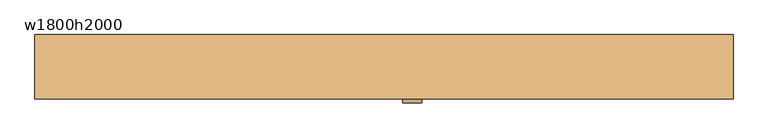
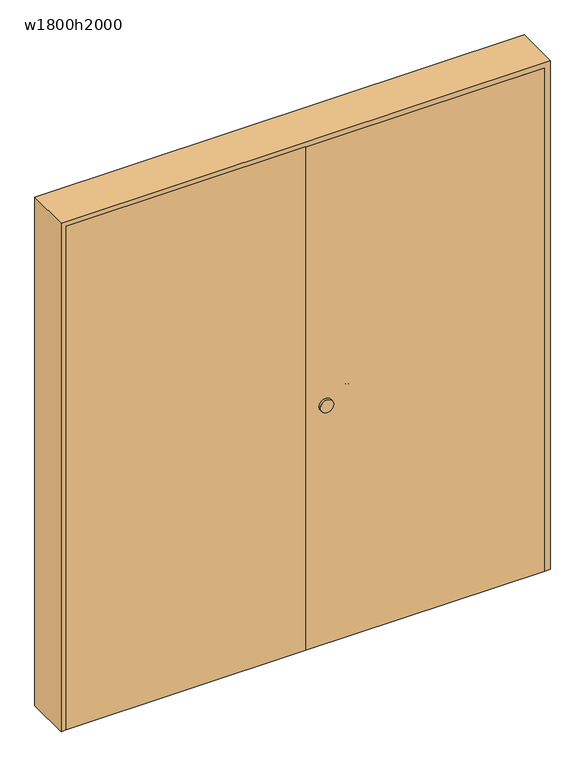
"""IFC4 building model written with IfcOpenShell, lengths in millimetres: door geometry, 二重 : w1800h2000."""

import ifcopenshell
import ifcopenshell.guid

model = None  # the IFC model being written
_history = None  # IfcOwnerHistory: only IFC2X3 demands one
_inside = {}  # id of a spatial element -> (the spatial element, [elements in it])
_under = {}  # id of a project, library or spatial element -> (it, [spatial elements below it])
_declared = {}  # id of a project -> (the project, [libraries it declares])
_typed = {}  # id of a type object -> (the type object, [elements of that type])
_made_of = {}  # id of a material, layer set ... -> (it, [elements and type objects made of it])


def new_model(schema):
    """Start an empty IFC model of exactly this schema.

    Asked for "IFC4X3", IfcOpenShell would pick the latest addendum, in which some entities
    have other attributes; the version numbers below select the first issue.
    IFC2X3 requires an IfcOwnerHistory on every rooted entity: one is made here for all.
    """
    global model, _history
    if schema == "IFC4X3":
        model = ifcopenshell.file(schema_version=(4, 3, 0, 0))
    else:
        model = ifcopenshell.file(schema=schema)
    _inside.clear()
    _under.clear()
    _declared.clear()
    _typed.clear()
    _made_of.clear()
    _history = None
    if model.schema == "IFC2X3":
        org = make("IfcOrganization", Name="unknown")
        user = make(
            "IfcPersonAndOrganization",
            ThePerson=make("IfcPerson", FamilyName="unknown"),
            TheOrganization=org,
        )
        app = make(
            "IfcApplication",
            ApplicationDeveloper=org,
            Version="unknown",
            ApplicationFullName="unknown",
            ApplicationIdentifier="unknown",
        )
        _history = make(
            "IfcOwnerHistory",
            OwningUser=user,
            OwningApplication=app,
            ChangeAction="ADDED",
            CreationDate=0,
        )
    return model


def make(cls, **values):
    """One entity of the class cls with the attributes given. An attribute that is None is left unset."""
    return model.create_entity(
        cls, **{name: value for name, value in values.items() if value is not None}
    )


def rooted(cls, **values):
    """An entity with a GlobalId (a new one), such as an element, a storey or a relation."""
    return make(cls, GlobalId=ifcopenshell.guid.new(), OwnerHistory=_history, **values)


def si_unit(unit_type, name, prefix=None):
    """IfcSIUnit, for example si_unit("LENGTHUNIT", "METRE", prefix="MILLI")."""
    return make("IfcSIUnit", UnitType=unit_type, Prefix=prefix, Name=name)


def assignment(units):
    """IfcUnitAssignment: the units of a project."""
    return None if units is None else make("IfcUnitAssignment", Units=units)


def point(xyz):
    """IfcCartesianPoint."""
    return None if xyz is None else make("IfcCartesianPoint", Coordinates=xyz)


def direction(xyz):
    """IfcDirection."""
    return None if xyz is None else make("IfcDirection", DirectionRatios=xyz)


def frame(location, z_axis=None, x_axis=None):
    """IfcAxis2Placement3D, a coordinate frame: its origin and axes. An axis left out is left unset."""
    return make(
        "IfcAxis2Placement3D",
        Location=point(location),
        Axis=direction(z_axis),
        RefDirection=direction(x_axis),
    )


def frame_2d(location, x_axis=None):
    """IfcAxis2Placement2D, a coordinate frame in the plane: its origin and x axis."""
    return make(
        "IfcAxis2Placement2D", Location=point(location), RefDirection=direction(x_axis)
    )


def origin():
    """The frame at (0, 0, 0) with its axes left unset."""
    return frame((0.0, 0.0, 0.0))


def origin_with_axes():
    """The frame at (0, 0, 0) with the z axis (0, 0, 1) and the x axis (1, 0, 0) written out."""
    return frame((0.0, 0.0, 0.0), z_axis=(0.0, 0.0, 1.0), x_axis=(1.0, 0.0, 0.0))


def place(relative_to, where):
    """IfcLocalPlacement: puts the frame where relative to a parent placement (None: the world)."""
    return make(
        "IfcLocalPlacement", PlacementRelTo=relative_to, RelativePlacement=where
    )


def context(
    kind, dimensions, precision=None, world=None, true_north=None, identifier=None
):
    """IfcGeometricRepresentationContext, for example the 3D "Model" context."""
    return make(
        "IfcGeometricRepresentationContext",
        ContextIdentifier=identifier,
        ContextType=kind,
        CoordinateSpaceDimension=dimensions,
        Precision=precision,
        WorldCoordinateSystem=world,
        TrueNorth=true_north,
    )


def project(units=None, contexts=None):
    """IfcProject with its units and contexts."""
    return rooted(
        "IfcProject",
        Name="project",
        RepresentationContexts=contexts,
        UnitsInContext=assignment(units),
    )


def spatial(cls, under=None, at=None, **own):
    """A site, building, storey or space (cls), placed at a placement, below another one or the project."""
    s = rooted(cls, ObjectPlacement=at, **own)
    if under is not None:
        _under.setdefault(under.id(), (under, []))[1].append(s)
    return s


def polyline(points):
    """IfcPolyline through the points."""
    return make("IfcPolyline", Points=[point(p) for p in points])


def circle_curve(where, radius):
    """IfcCircle in the frame where."""
    return make("IfcCircle", Position=where, Radius=radius)


def ellipse_curve(where, semi_axis1, semi_axis2):
    """IfcEllipse in the frame where."""
    return make(
        "IfcEllipse", Position=where, SemiAxis1=semi_axis1, SemiAxis2=semi_axis2
    )


def trimmed(basis, trim1, trim2, sense, master):
    """IfcTrimmedCurve: the piece of a basis curve between two trims."""
    return make(
        "IfcTrimmedCurve",
        BasisCurve=basis,
        Trim1=trim1,
        Trim2=trim2,
        SenseAgreement=sense,
        MasterRepresentation=master,
    )


def segment(curve, same_sense, transition):
    """IfcCompositeCurveSegment."""
    return make(
        "IfcCompositeCurveSegment",
        Transition=transition,
        SameSense=same_sense,
        ParentCurve=curve,
    )


def composite_curve(segments, self_intersect=None):
    """IfcCompositeCurve: segments joined end to end."""
    return make("IfcCompositeCurve", Segments=segments, SelfIntersect=self_intersect)


def outline(outer, holes=None, kind="AREA"):
    """IfcArbitraryClosedProfileDef: a profile drawn as a closed curve; with holes, ...WithVoids."""
    if holes is None:
        return make("IfcArbitraryClosedProfileDef", ProfileType=kind, OuterCurve=outer)
    return make(
        "IfcArbitraryProfileDefWithVoids",
        ProfileType=kind,
        OuterCurve=outer,
        InnerCurves=holes,
    )


def extrude(swept, where, along, depth):
    """IfcExtrudedAreaSolid: the profile swept, set in the frame where, extruded along a direction by depth."""
    return make(
        "IfcExtrudedAreaSolid",
        SweptArea=swept,
        Position=where,
        ExtrudedDirection=direction(along),
        Depth=depth,
    )


def shape(context_of_items, identifier, shape_type, items):
    """IfcShapeRepresentation: the items that make up one representation, for example the "Body"."""
    return make(
        "IfcShapeRepresentation",
        ContextOfItems=context_of_items,
        RepresentationIdentifier=identifier,
        RepresentationType=shape_type,
        Items=items,
    )


def source(mapping_origin, context_of_items, identifier, shape_type, items):
    """IfcRepresentationMap: a shape defined once, which mapped items show again and again."""
    return make(
        "IfcRepresentationMap",
        MappingOrigin=mapping_origin,
        MappedRepresentation=shape(context_of_items, identifier, shape_type, items),
    )


def transform(
    local_origin,
    x_axis=None,
    y_axis=None,
    z_axis=None,
    scale=None,
    scale2=None,
    scale3=None,
    uniform=True,
):
    """IfcCartesianTransformationOperator3D, or its non-uniform kind. x_axis, y_axis, z_axis: its Axis1, 2, 3."""
    if uniform:
        return make(
            "IfcCartesianTransformationOperator3D",
            Axis1=direction(x_axis),
            Axis2=direction(y_axis),
            LocalOrigin=point(local_origin),
            Scale=scale,
            Axis3=direction(z_axis),
        )
    return make(
        "IfcCartesianTransformationOperator3DnonUniform",
        Axis1=direction(x_axis),
        Axis2=direction(y_axis),
        LocalOrigin=point(local_origin),
        Scale=scale,
        Axis3=direction(z_axis),
        Scale2=scale2,
        Scale3=scale3,
    )


def mapped(mapping_source, mapping_target):
    """IfcMappedItem: shows the shape of a source again, moved by a transform."""
    return make(
        "IfcMappedItem", MappingSource=mapping_source, MappingTarget=mapping_target
    )


def made_of(thing, what):
    """Note that an element or type object is made of a material, layer set ...; save() writes the relation."""
    if what is not None:
        _made_of.setdefault(what.id(), (what, []))[1].append(thing)
    return thing


def element(
    cls,
    number,
    at=None,
    inside=None,
    cuts=None,
    type_object=None,
    material=None,
    context=None,
    identifier="Body",
    shape_type=None,
    held_by="IfcProductDefinitionShape",
    body=None,
    shapes=None,
    **own,
):
    """One element of the class cls, such as IfcWall. Its Tag is "e" and its number.

    at: its placement. inside: the storey or other place that contains it. cuts: it is an
    opening in that element (IfcRelVoidsElement). A single representation is given by context,
    identifier, shape_type and body (its items); several are given by shapes. held_by: the class
    of the entity that holds the representations. save() writes the other relations.
    """
    e = rooted(cls, Tag="e%d" % number, ObjectPlacement=at, **own)
    if body is not None:
        shapes = [shape(context, identifier, shape_type, body)]
    if shapes is not None:
        e.Representation = make(held_by, Representations=shapes)
    if inside is not None:
        _inside.setdefault(inside.id(), (inside, []))[1].append(e)
    if cuts is not None:
        rooted(
            "IfcRelVoidsElement", RelatingBuildingElement=cuts, RelatedOpeningElement=e
        )
    if type_object is not None:
        _typed.setdefault(type_object.id(), (type_object, []))[1].append(e)
    return made_of(e, material)


def aggregate(whole, parts):
    """IfcRelAggregates: a whole, such as a stair, and the parts it consists of."""
    return rooted("IfcRelAggregates", RelatingObject=whole, RelatedObjects=parts)


def save(model, path):
    """Write the relations noted so far, then the file.

    IfcRelAggregates (storeys below a building ...), IfcRelContainedInSpatialStructure (elements
    in a storey), IfcRelDefinesByType, IfcRelAssociatesMaterial and IfcRelDeclares: one each for
    every whole, place, type object, material and project.
    """
    for whole, parts in _under.values():
        aggregate(whole, parts)
    for where, things in _inside.values():
        rooted(
            "IfcRelContainedInSpatialStructure",
            RelatedElements=things,
            RelatingStructure=where,
        )
    for kind, things in _typed.values():
        rooted("IfcRelDefinesByType", RelatedObjects=things, RelatingType=kind)
    for what, things in _made_of.values():
        rooted("IfcRelAssociatesMaterial", RelatedObjects=things, RelatingMaterial=what)
    for by, libraries in _declared.values():
        rooted("IfcRelDeclares", RelatingContext=by, RelatedDefinitions=libraries)
    model.write(path)


def plane_surface(at):
    """IfcPlane: the flat surface through the origin of the frame at, square to its z axis."""
    return make("IfcPlane", Position=at)


def cylinder_surface(at, radius):
    """IfcCylindricalSurface: all points at the distance radius from the z axis of the frame at."""
    return make("IfcCylindricalSurface", Position=at, Radius=radius)


def revolved_surface(curve, axis_point, axis_direction):
    """IfcSurfaceOfRevolution: the curve turned about the line through axis_point along axis_direction."""
    return make(
        "IfcSurfaceOfRevolution",
        SweptCurve=make("IfcArbitraryOpenProfileDef", ProfileType="CURVE", Curve=curve),
        AxisPosition=make("IfcAxis1Placement", Location=point(axis_point), Axis=direction(axis_direction)),
    )


def advanced_brep(points, edges, surfaces, faces):
    """IfcAdvancedBrep: a solid bounded by faces that lie on surfaces and meet in shared edges.

    An edge is (start, end): straight between two places in points (the first is 0);
    or (start, end, curve); or (start, end, curve, False) where it runs against its curve.
    A face is (place in surfaces, loops), or (place, loops, False) where it looks against
    its surface's normal. A loop lists edges by number (the first is 1), with a minus sign
    where the edge is run from its end to its start. The first loop is the outer one.
    """
    corners = [point(p) for p in points]
    vertices = [make("IfcVertexPoint", VertexGeometry=c) for c in corners]
    made = []
    for start, end, *more in edges:
        made.append(
            make(
                "IfcEdgeCurve",
                EdgeStart=vertices[start],
                EdgeEnd=vertices[end],
                EdgeGeometry=more[0] if more else make("IfcPolyline", Points=[corners[start], corners[end]]),
                SameSense=more[1] if len(more) > 1 else True,
            )
        )
    hull = []
    for where, loops, *sense in faces:
        bounds = []
        for j, loop in enumerate(loops):
            ring = [make("IfcOrientedEdge", EdgeElement=made[abs(k) - 1], Orientation=k > 0) for k in loop]
            bounds.append(
                make(
                    "IfcFaceOuterBound" if j == 0 else "IfcFaceBound",
                    Bound=make("IfcEdgeLoop", EdgeList=ring),
                    Orientation=True,
                )
            )
        hull.append(make("IfcAdvancedFace", Bounds=bounds, FaceSurface=surfaces[where], SameSense=sense[0] if sense else True))
    return make("IfcAdvancedBrep", Outer=make("IfcClosedShell", CfsFaces=hull))


def w1800h2000_e7756d22(model_context):
    return source(origin(), model_context, "Body", "SolidModel", [
        advanced_brep(
        [(77.0, -45.0, 940.0), (82.0, -45.0, 945.0), (82.0, -45.0, 955.0), (77.0, -45.0, 960.0), (73.0, -45.0, 960.0), (68.0, -45.0, 955.0), (68.0, -45.0, 945.0), (73.0, -45.0, 940.0), (73.0, -10.0, 940.0), (85.0, 2.0, 940.0), (200.0, 2.0, 940.0), (212.0, -10.0, 940.0), (212.0, -15.0, 940.0), (208.0, -15.0, 940.0), (208.0, -10.0, 940.0), (200.0, -2.0, 940.0), (85.0, -2.0, 940.0), (77.0, -10.0, 940.0), (68.0, -10.0, 945.0), (68.0, -10.0, 955.0), (73.0, -10.0, 960.0), (77.0, -10.0, 960.0), (85.0, -2.0, 960.0), (200.0, -2.0, 960.0), (208.0, -10.0, 960.0), (208.0, -15.0, 960.0), (212.0, -15.0, 960.0), (212.0, -10.0, 960.0), (200.0, 2.0, 960.0), (85.0, 2.0, 960.0), (82.0, -10.0, 955.0), (82.0, -10.0, 945.0), (85.0, 7.0, 945.0), (85.0, 7.0, 955.0), (85.0, -7.0, 955.0), (85.0, -7.0, 945.0), (200.0, 7.0, 945.0), (200.0, 7.0, 955.0), (200.0, -7.0, 955.0), (200.0, -7.0, 945.0), (217.0, -10.0, 945.0), (217.0, -10.0, 955.0), (203.0, -10.0, 955.0), (203.0, -10.0, 945.0), (217.0, -15.0, 945.0), (217.0, -15.0, 955.0), (203.0, -15.0, 955.0), (203.0, -15.0, 945.0)],
        [
            (0, 1, circle_curve(frame((77.0, -45.0, 945.0), z_axis=(0.0, -1.0, 0.0), x_axis=(1.0, 0.0, 0.0)), 5.0)),
            (1, 2),
            (2, 3, circle_curve(frame((77.0, -45.0, 955.0), z_axis=(0.0, -1.0, 0.0), x_axis=(1.0, 0.0, 0.0)), 5.0)),
            (3, 4),
            (4, 5, circle_curve(frame((73.0, -45.0, 955.0), z_axis=(0.0, -1.0, 0.0), x_axis=(1.0, 0.0, 0.0)), 5.0)),
            (5, 6),
            (6, 7, circle_curve(frame((73.0, -45.0, 945.0), z_axis=(0.0, -1.0, 0.0), x_axis=(1.0, 0.0, 0.0)), 5.0)),
            (7, 0),
            (7, 8),
            (8, 9, circle_curve(frame((85.0, -10.0, 940.0), z_axis=(0.0, 0.0, -1.0), x_axis=(-1.0, 0.0, 0.0)), 12.0)),
            (9, 10),
            (10, 11, circle_curve(frame((200.0, -10.0, 940.0), z_axis=(0.0, 0.0, -1.0), x_axis=(0.0, 1.0, 0.0)), 12.0)),
            (11, 12),
            (12, 13),
            (13, 14),
            (14, 15, circle_curve(frame((200.0, -10.0, 940.0), z_axis=(0.0, 0.0, 1.0), x_axis=(0.0, 1.0, 0.0)), 8.0)),
            (15, 16),
            (16, 17, circle_curve(frame((85.0, -10.0, 940.0), z_axis=(0.0, 0.0, 1.0), x_axis=(-1.0, 0.0, 0.0)), 8.0)),
            (17, 0),
            (6, 18),
            (18, 8, circle_curve(frame((73.0, -10.0, 945.0), z_axis=(0.0, -1.0, 0.0), x_axis=(1.0, 0.0, 0.0)), 5.0)),
            (5, 19),
            (19, 18),
            (4, 20),
            (20, 19, circle_curve(frame((73.0, -10.0, 955.0), z_axis=(0.0, -1.0, 0.0), x_axis=(1.0, 0.0, 0.0)), 5.0)),
            (3, 21),
            (21, 22, circle_curve(frame((85.0, -10.0, 960.0), z_axis=(0.0, 0.0, -1.0), x_axis=(-1.0, 0.0, 0.0)), 8.0)),
            (22, 23),
            (23, 24, circle_curve(frame((200.0, -10.0, 960.0), z_axis=(0.0, 0.0, -1.0), x_axis=(0.0, 1.0, 0.0)), 8.0)),
            (24, 25),
            (25, 26),
            (26, 27),
            (27, 28, circle_curve(frame((200.0, -10.0, 960.0), z_axis=(0.0, 0.0, 1.0), x_axis=(0.0, 1.0, 0.0)), 12.0)),
            (28, 29),
            (29, 20, circle_curve(frame((85.0, -10.0, 960.0), z_axis=(0.0, 0.0, 1.0), x_axis=(-1.0, 0.0, 0.0)), 12.0)),
            (2, 30),
            (30, 21, circle_curve(frame((77.0, -10.0, 955.0), z_axis=(0.0, -1.0, 0.0), x_axis=(1.0, 0.0, 0.0)), 5.0)),
            (1, 31),
            (31, 30),
            (17, 31, circle_curve(frame((77.0, -10.0, 945.0), z_axis=(0.0, -1.0, 0.0), x_axis=(1.0, 0.0, 0.0)), 5.0)),
            (32, 9, circle_curve(frame((85.0, 2.0, 945.0), z_axis=(-1.0, 0.0, 0.0), x_axis=(0.0, -1.0, 0.0)), 5.0)),
            (18, 32, circle_curve(frame((85.0, -10.0, 945.0), z_axis=(0.0, 0.0, -1.0), x_axis=(-1.0, 0.0, 0.0)), 17.0)),
            (33, 32),
            (19, 33, circle_curve(frame((85.0, -10.0, 955.0), z_axis=(0.0, 0.0, -1.0), x_axis=(-1.0, 0.0, 0.0)), 17.0)),
            (29, 33, circle_curve(frame((85.0, 2.0, 955.0), z_axis=(-1.0, 0.0, 0.0), x_axis=(0.0, -1.0, 0.0)), 5.0)),
            (34, 22, circle_curve(frame((85.0, -2.0, 955.0), z_axis=(-1.0, 0.0, 0.0), x_axis=(0.0, -1.0, 0.0)), 5.0)),
            (30, 34, circle_curve(frame((85.0, -10.0, 955.0), z_axis=(0.0, 0.0, -1.0), x_axis=(-1.0, 0.0, 0.0)), 3.0)),
            (35, 34),
            (31, 35, circle_curve(frame((85.0, -10.0, 945.0), z_axis=(0.0, 0.0, -1.0), x_axis=(-1.0, 0.0, 0.0)), 3.0)),
            (16, 35, circle_curve(frame((85.0, -2.0, 945.0), z_axis=(-1.0, 0.0, 0.0), x_axis=(0.0, -1.0, 0.0)), 5.0)),
            (32, 36),
            (36, 10, circle_curve(frame((200.0, 2.0, 945.0), z_axis=(-1.0, 0.0, 0.0), x_axis=(0.0, -1.0, 0.0)), 5.0)),
            (33, 37),
            (37, 36),
            (28, 37, circle_curve(frame((200.0, 2.0, 955.0), z_axis=(-1.0, 0.0, 0.0), x_axis=(0.0, -1.0, 0.0)), 5.0)),
            (34, 38),
            (38, 23, circle_curve(frame((200.0, -2.0, 955.0), z_axis=(-1.0, 0.0, 0.0), x_axis=(0.0, -1.0, 0.0)), 5.0)),
            (35, 39),
            (39, 38),
            (15, 39, circle_curve(frame((200.0, -2.0, 945.0), z_axis=(-1.0, 0.0, 0.0), x_axis=(0.0, -1.0, 0.0)), 5.0)),
            (40, 11, circle_curve(frame((212.0, -10.0, 945.0), z_axis=(0.0, 1.0, 0.0), x_axis=(-1.0, 0.0, 0.0)), 5.0)),
            (36, 40, circle_curve(frame((200.0, -10.0, 945.0), z_axis=(0.0, 0.0, -1.0), x_axis=(0.0, 1.0, 0.0)), 17.0)),
            (41, 40),
            (37, 41, circle_curve(frame((200.0, -10.0, 955.0), z_axis=(0.0, 0.0, -1.0), x_axis=(0.0, 1.0, 0.0)), 17.0)),
            (27, 41, circle_curve(frame((212.0, -10.0, 955.0), z_axis=(0.0, 1.0, 0.0), x_axis=(-1.0, 0.0, 0.0)), 5.0)),
            (42, 24, circle_curve(frame((208.0, -10.0, 955.0), z_axis=(0.0, 1.0, 0.0), x_axis=(-1.0, 0.0, 0.0)), 5.0)),
            (38, 42, circle_curve(frame((200.0, -10.0, 955.0), z_axis=(0.0, 0.0, -1.0), x_axis=(0.0, 1.0, 0.0)), 3.0)),
            (43, 42),
            (39, 43, circle_curve(frame((200.0, -10.0, 945.0), z_axis=(0.0, 0.0, -1.0), x_axis=(0.0, 1.0, 0.0)), 3.0)),
            (14, 43, circle_curve(frame((208.0, -10.0, 945.0), z_axis=(0.0, 1.0, 0.0), x_axis=(-1.0, 0.0, 0.0)), 5.0)),
            (12, 44, circle_curve(frame((212.0, -15.0, 945.0), z_axis=(0.0, -1.0, 0.0), x_axis=(-1.0, 0.0, 0.0)), 5.0)),
            (44, 45),
            (45, 26, circle_curve(frame((212.0, -15.0, 955.0), z_axis=(0.0, -1.0, 0.0), x_axis=(-1.0, 0.0, 0.0)), 5.0)),
            (25, 46, circle_curve(frame((208.0, -15.0, 955.0), z_axis=(0.0, -1.0, 0.0), x_axis=(-1.0, 0.0, 0.0)), 5.0)),
            (46, 47),
            (47, 13, circle_curve(frame((208.0, -15.0, 945.0), z_axis=(0.0, -1.0, 0.0), x_axis=(-1.0, 0.0, 0.0)), 5.0)),
            (40, 44),
            (41, 45),
            (42, 46),
            (43, 47),
        ],
        [
            plane_surface(frame((64.801961, -45.0, 950.0), z_axis=(0.0, -1.0, 0.0), x_axis=(0.0, 0.0, -1.0))),
            plane_surface(frame((77.0, -45.0, 940.0), z_axis=(0.0, 0.0, -1.0), x_axis=(0.0, 1.0, 0.0))),
            cylinder_surface(frame((73.0, -45.0, 945.0), z_axis=(0.0, -1.0, 0.0), x_axis=(1.0, 0.0, 0.0)), 5.0),
            plane_surface(frame((68.0, -45.0, 945.0), z_axis=(-1.0, 0.0, 0.0), x_axis=(0.0, 1.0, 0.0))),
            cylinder_surface(frame((73.0, -45.0, 955.0), z_axis=(0.0, -1.0, 0.0), x_axis=(1.0, 0.0, 0.0)), 5.0),
            plane_surface(frame((73.0, -45.0, 960.0), z_axis=(0.0, 0.0, 1.0), x_axis=(0.0, 1.0, 0.0))),
            cylinder_surface(frame((77.0, -45.0, 955.0), z_axis=(0.0, -1.0, 0.0), x_axis=(1.0, 0.0, 0.0)), 5.0),
            plane_surface(frame((82.0, -45.0, 955.0), z_axis=(1.0, 0.0, 0.0), x_axis=(0.0, 1.0, 0.0))),
            cylinder_surface(frame((77.0, -45.0, 945.0), z_axis=(0.0, -1.0, 0.0), x_axis=(1.0, 0.0, 0.0)), 5.0),
            revolved_surface(trimmed(ellipse_curve(frame((73.0, -10.0, 945.0), z_axis=(0.0, 1.0, 0.0), x_axis=(1.0, 0.0, 0.0)), 5.0, 5.0), [point((73.0, -10.0, 940.0))], [point((68.0, -10.0, 945.0))], True, "CARTESIAN"), (85.0, -10.0, 950.0), (0.0, 0.0, 1.0)),
            cylinder_surface(frame((85.0, -10.0, 950.0), z_axis=(0.0, 0.0, 1.0), x_axis=(-1.0, 0.0, 0.0)), 17.0),
            revolved_surface(trimmed(ellipse_curve(frame((73.0, -10.0, 955.0), z_axis=(0.0, 1.0, 0.0), x_axis=(1.0, 0.0, 0.0)), 5.0, 5.0), [point((68.0, -10.0, 955.0))], [point((73.0, -10.0, 960.0))], True, "CARTESIAN"), (85.0, -10.0, 950.0), (0.0, 0.0, 1.0)),
            revolved_surface(trimmed(ellipse_curve(frame((77.0, -10.0, 955.0), z_axis=(0.0, 1.0, 0.0), x_axis=(1.0, 0.0, 0.0)), 5.0, 5.0), [point((77.0, -10.0, 960.0))], [point((82.0, -10.0, 955.0))], True, "CARTESIAN"), (85.0, -10.0, 950.0), (0.0, 0.0, 1.0)),
            revolved_surface(polyline([(82.0, -10.0, 955.0), (82.0, -10.0, 945.0)]), (85.0, -10.0, 950.0), (0.0, 0.0, 1.0)),
            revolved_surface(trimmed(ellipse_curve(frame((77.0, -10.0, 945.0), z_axis=(0.0, 1.0, 0.0), x_axis=(1.0, 0.0, 0.0)), 5.0, 5.0), [point((82.0, -10.0, 945.0))], [point((77.0, -10.0, 940.0))], True, "CARTESIAN"), (85.0, -10.0, 950.0), (0.0, 0.0, 1.0)),
            cylinder_surface(frame((85.0, 2.0, 945.0), z_axis=(-1.0, 0.0, 0.0), x_axis=(0.0, -1.0, 0.0)), 5.0),
            plane_surface(frame((85.0, 7.0, 945.0), z_axis=(0.0, 1.0, 0.0), x_axis=(1.0, 0.0, 0.0))),
            cylinder_surface(frame((85.0, 2.0, 955.0), z_axis=(-1.0, 0.0, 0.0), x_axis=(0.0, -1.0, 0.0)), 5.0),
            cylinder_surface(frame((85.0, -2.0, 955.0), z_axis=(-1.0, 0.0, 0.0), x_axis=(0.0, -1.0, 0.0)), 5.0),
            plane_surface(frame((85.0, -7.0, 955.0), z_axis=(0.0, -1.0, 0.0), x_axis=(1.0, 0.0, 0.0))),
            cylinder_surface(frame((85.0, -2.0, 945.0), z_axis=(-1.0, 0.0, 0.0), x_axis=(0.0, -1.0, 0.0)), 5.0),
            revolved_surface(trimmed(ellipse_curve(frame((200.0, 2.0, 945.0), z_axis=(1.0, 0.0, 0.0), x_axis=(0.0, -1.0, 0.0)), 5.0, 5.0), [point((200.0, 2.0, 940.0))], [point((200.0, 7.0, 945.0))], True, "CARTESIAN"), (200.0, -10.0, 950.0), (0.0, 0.0, 1.0)),
            cylinder_surface(frame((200.0, -10.0, 950.0), z_axis=(0.0, 0.0, 1.0), x_axis=(0.0, 1.0, 0.0)), 17.0),
            revolved_surface(trimmed(ellipse_curve(frame((200.0, 2.0, 955.0), z_axis=(1.0, 0.0, 0.0), x_axis=(0.0, -1.0, 0.0)), 5.0, 5.0), [point((200.0, 7.0, 955.0))], [point((200.0, 2.0, 960.0))], True, "CARTESIAN"), (200.0, -10.0, 950.0), (0.0, 0.0, 1.0)),
            revolved_surface(trimmed(ellipse_curve(frame((200.0, -2.0, 955.0), z_axis=(1.0, 0.0, 0.0), x_axis=(0.0, -1.0, 0.0)), 5.0, 5.0), [point((200.0, -2.0, 960.0))], [point((200.0, -7.0, 955.0))], True, "CARTESIAN"), (200.0, -10.0, 950.0), (0.0, 0.0, 1.0)),
            revolved_surface(polyline([(200.0, -7.0, 955.0), (200.0, -7.0, 945.0)]), (200.0, -10.0, 950.0), (0.0, 0.0, 1.0)),
            revolved_surface(trimmed(ellipse_curve(frame((200.0, -2.0, 945.0), z_axis=(1.0, 0.0, 0.0), x_axis=(0.0, -1.0, 0.0)), 5.0, 5.0), [point((200.0, -7.0, 945.0))], [point((200.0, -2.0, 940.0))], True, "CARTESIAN"), (200.0, -10.0, 950.0), (0.0, 0.0, 1.0)),
            plane_surface(frame((199.801961, -15.0, 950.0), z_axis=(0.0, -1.0, 0.0), x_axis=(0.0, 0.0, 1.0))),
            cylinder_surface(frame((212.0, -10.0, 945.0), z_axis=(0.0, 1.0, 0.0), x_axis=(-1.0, 0.0, 0.0)), 5.0),
            plane_surface(frame((217.0, -10.0, 945.0), z_axis=(1.0, 0.0, 0.0), x_axis=(0.0, -1.0, 0.0))),
            cylinder_surface(frame((212.0, -10.0, 955.0), z_axis=(0.0, 1.0, 0.0), x_axis=(-1.0, 0.0, 0.0)), 5.0),
            cylinder_surface(frame((208.0, -10.0, 955.0), z_axis=(0.0, 1.0, 0.0), x_axis=(-1.0, 0.0, 0.0)), 5.0),
            plane_surface(frame((203.0, -10.0, 955.0), z_axis=(-1.0, 0.0, 0.0), x_axis=(0.0, -1.0, 0.0))),
            cylinder_surface(frame((208.0, -10.0, 945.0), z_axis=(0.0, 1.0, 0.0), x_axis=(-1.0, 0.0, 0.0)), 5.0),
        ],
        [
            (0, [[1, 2, 3, 4, 5, 6, 7, 8]]),
            (1, [[9, 10, 11, 12, 13, 14, 15, 16, 17, 18, 19, -8]]),
            (2, [[20, 21, -9, -7]]),
            (3, [[22, 23, -20, -6]]),
            (4, [[24, 25, -22, -5]]),
            (5, [[26, 27, 28, 29, 30, 31, 32, 33, 34, 35, -24, -4]]),
            (6, [[36, 37, -26, -3]]),
            (7, [[38, 39, -36, -2]]),
            (8, [[-19, 40, -38, -1]]),
            (9, [[41, -10, -21, 42]]),
            (10, [[43, -42, -23, 44]]),
            (11, [[45, -44, -25, -35]]),
            (12, [[46, -27, -37, 47]]),
            (13, [[48, -47, -39, 49]]),
            (14, [[50, -49, -40, -18]]),
            (15, [[51, 52, -11, -41]]),
            (16, [[53, 54, -51, -43]]),
            (17, [[-34, 55, -53, -45]]),
            (18, [[56, 57, -28, -46]]),
            (19, [[58, 59, -56, -48]]),
            (20, [[-17, 60, -58, -50]]),
            (21, [[61, -12, -52, 62]]),
            (22, [[63, -62, -54, 64]]),
            (23, [[65, -64, -55, -33]]),
            (24, [[66, -29, -57, 67]]),
            (25, [[68, -67, -59, 69]]),
            (26, [[70, -69, -60, -16]]),
            (27, [[-14, 71, 72, 73, -31, 74, 75, 76]]),
            (28, [[77, -71, -13, -61]]),
            (29, [[78, -72, -77, -63]]),
            (30, [[-32, -73, -78, -65]]),
            (31, [[79, -74, -30, -66]]),
            (32, [[80, -75, -79, -68]]),
            (33, [[-15, -76, -80, -70]]),
        ],
    ),
        extrude(outline(composite_curve([segment(trimmed(circle_curve(frame_2d((950.0, 75.0)), 25.0), [point((950.0, 50.0))], [point((950.0, 100.0))], False, "CARTESIAN"), True, "CONTINUOUS"), segment(trimmed(circle_curve(frame_2d((950.0, 75.0)), 25.0), [point((950.0, 100.0))], [point((950.0, 50.0))], False, "CARTESIAN"), True, "CONTINUOUS")], self_intersect=False)), frame((0.0, -95.0, 0.0), z_axis=(0.0, 1.0, 0.0), x_axis=(0.0, 0.0, 1.0)), (0.0, 0.0, 1.0), 10.0),
        extrude(outline(composite_curve([segment(trimmed(circle_curve(frame_2d((950.0, 75.0)), 25.0), [point((950.0, 50.0))], [point((950.0, 100.0))], False, "CARTESIAN"), True, "CONTINUOUS"), segment(trimmed(circle_curve(frame_2d((950.0, 75.0)), 25.0), [point((950.0, 100.0))], [point((950.0, 50.0))], False, "CARTESIAN"), True, "CONTINUOUS")], self_intersect=False)), frame((0.0, -55.0, 0.0), z_axis=(0.0, 1.0, 0.0), x_axis=(0.0, 0.0, 1.0)), (0.0, 0.0, 1.0), 10.0),
        extrude(outline(polyline([(0.0, -55.0), (0.0, -85.0), (-900.0, -85.0), (-900.0, -55.0), (0.0, -55.0)])), origin_with_axes(), (0.0, 0.0, 1.0), 2000.0),
        extrude(outline(polyline([(2020.0, -920.0), (0.0, -920.0), (0.0, -900.0), (2000.0, -900.0), (2000.0, 900.0), (0.0, 900.0), (0.0, 920.0), (2020.0, 920.0), (2020.0, -920.0)])), frame((0.0, -85.0, 0.0), z_axis=(0.0, 1.0, 0.0), x_axis=(0.0, 0.0, 1.0)), (0.0, 0.0, 1.0), 170.0),
        extrude(outline(polyline([(900.0, -55.0), (900.0, -85.0), (0.0, -85.0), (0.0, -55.0), (900.0, -55.0)])), origin_with_axes(), (0.0, 0.0, 1.0), 2000.0),
    ])


if __name__ == "__main__":
    model = new_model("IFC4")
    model_context = context("Model", 3, world=origin())
    ifc_project = project(units=[si_unit("LENGTHUNIT", "METRE", prefix="MILLI")], contexts=[model_context])
    site = spatial("IfcSite", under=ifc_project)
    building = spatial("IfcBuilding", under=site)
    placement = place(None, origin())
    w1800h2000_shape = w1800h2000_e7756d22(model_context)
    element("IfcDoor", 1, ObjectType="二重 : w1800h2000", at=placement, inside=building, context=model_context, shape_type="MappedRepresentation", body=[
        mapped(w1800h2000_shape, transform((0.0, 0.0, 0.0), x_axis=(1.0, 0.0, 0.0), y_axis=(0.0, 1.0, 0.0), z_axis=(0.0, 0.0, 1.0))),
    ])
    save(model, "model.ifc")

# Revit data of these elements
# Type "二重 : w1800h2000"
#   Construction Type Id = "MDOOR"
#   Analytic Construction = "メタル"
#   Type Mark = "45"
#   Operation = "両開きドア単一スイング"
#   Keynote = "08110.R1"
#   Visual Light Transmittance = 0
#   Solar Heat Gain Coefficient = 0
#   Heat Transfer Coefficient (U) = 3.7021 W/(m²·K)
#   高さ(中心) = 1000 mm
#   Height = 2000 mm
#   Thickness = 30 mm
#   ドア枠見附 = 20 mm
#   Width = 1800 mm
#   取手取付け高さ = 950 mm
#   ドア枠ちり = 10 mm
#   Function = 0
#   ドア枠 [instance default] = none
#   ドア把手 [instance default] = メタル-ステンレス
#   ドア [instance default] = none
#   Wall Closure = (empty or 0)
# Element 1 (IfcDoor, "二重 : w1800h2000")
#   Materials on its faces: "メタル-ステンレス"
# Materials
#   "メタル-ステンレス": class "メタル", colour RGB 247 247 247, transparency 0, Cost = 0
